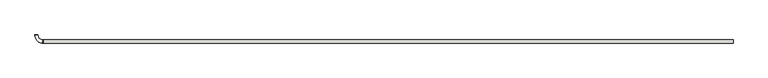
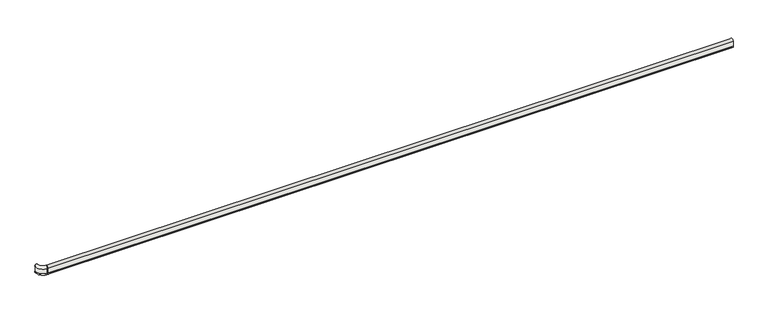
"""IFC4 building model written with IfcOpenShell, lengths in millimetres: covering geometry, Construction_Railing_SPM_Starline-Anodisee-Decowood : Decowood."""

from ifc_helpers import new_model, si_unit, point, frame, frame_2d, origin, place, context, project, spatial, polyline, circle_curve, ellipse_curve, trimmed, segment, composite_curve, outline, extrude, source, transform, mapped, element, save
from ifc_brep_helpers import plane_surface, cylinder_surface, revolved_surface, advanced_brep


def covering_4a841b85(model_context):
    return source(origin(), model_context, "Body", "SolidModel", [
        advanced_brep(
        [(0.0, -52.1949146, 777.1298269), (0.0, -78.97282, 779.8387167), (0.0, -77.7797808, 779.8387167), (0.0, -77.7797808, 730.187687), (0.0, -79.0444967, 730.187687), (0.0, -52.1949146, 732.7970729), (-1.0, -52.1949146, 777.1298269), (-1.0, -78.97282, 779.8387167), (-78.97282, -1.0, 779.8387167), (-78.97282, 0.0, 779.8387167), (-77.7797808, 0.0, 779.8387167), (-77.7797808, -1.0, 779.8387167), (-1.0, -77.7797808, 779.8387167), (-1.0, -77.7797808, 730.187687), (-77.7797808, -1.0, 730.187687), (-77.7797808, 0.0, 730.187687), (-79.0444967, 0.0, 730.187687), (-79.0444967, -1.0, 730.187687), (-1.0, -79.0444967, 730.187687), (-1.0, -52.1949146, 732.7970729), (-52.1949146, -1.0, 777.1298269), (-52.1949146, -1.0, 732.7970729), (-52.1949146, 0.0, 777.1298269), (-52.1949146, 0.0, 732.7970729)],
        [
            (0, 1, circle_curve(frame((0.0, -64.921376, 785.0331273), z_axis=(1.0, 0.0, 0.0), x_axis=(0.0, -1.0, 0.0)), 14.9808204)),
            (1, 2),
            (2, 3),
            (3, 4),
            (4, 5, circle_curve(frame((0.0, -64.9833199, 724.9442146), z_axis=(1.0, 0.0, 0.0), x_axis=(0.0, -1.0, 0.0)), 15.0070215)),
            (5, 0),
            (0, 6),
            (6, 7, circle_curve(frame((-1.0, -64.921376, 785.0331273), z_axis=(1.0, 0.0, 0.0), x_axis=(0.0, -1.0, 0.0)), 14.9808204)),
            (7, 1),
            (7, 8, circle_curve(frame((-1.0, -1.0, 779.8387167), z_axis=(0.0, 0.0, -1.0), x_axis=(0.0, -1.0, 0.0)), 77.97282)),
            (8, 9),
            (9, 10),
            (10, 11),
            (11, 12, circle_curve(frame((-1.0, -1.0, 779.8387167), z_axis=(0.0, 0.0, 1.0), x_axis=(0.0, -1.0, 0.0)), 76.7797808)),
            (12, 2),
            (12, 13),
            (13, 3),
            (13, 14, circle_curve(frame((-1.0, -1.0, 730.187687), z_axis=(0.0, 0.0, -1.0), x_axis=(0.0, -1.0, 0.0)), 76.7797808)),
            (14, 15),
            (15, 16),
            (16, 17),
            (17, 18, circle_curve(frame((-1.0, -1.0, 730.187687), z_axis=(0.0, 0.0, 1.0), x_axis=(0.0, -1.0, 0.0)), 78.0444967)),
            (18, 4),
            (18, 19, circle_curve(frame((-1.0, -64.9833199, 724.9442146), z_axis=(1.0, 0.0, 0.0), x_axis=(0.0, -1.0, 0.0)), 15.0070215)),
            (19, 5),
            (19, 6),
            (6, 20, circle_curve(frame((-1.0, -1.0, 777.1298269), z_axis=(0.0, 0.0, -1.0), x_axis=(0.0, -1.0, 0.0)), 51.1949146)),
            (20, 8, circle_curve(frame((-64.921376, -1.0, 785.0331273), z_axis=(0.0, -1.0, 0.0), x_axis=(-1.0, 0.0, 0.0)), 14.9808204)),
            (11, 14),
            (21, 19, circle_curve(frame((-1.0, -1.0, 732.7970729), z_axis=(0.0, 0.0, 1.0), x_axis=(0.0, -1.0, 0.0)), 51.1949146)),
            (17, 21, circle_curve(frame((-64.9833199, -1.0, 724.9442146), z_axis=(0.0, -1.0, 0.0), x_axis=(-1.0, 0.0, 0.0)), 15.0070215)),
            (21, 20),
            (22, 23),
            (23, 16, circle_curve(frame((-64.9833199, 0.0, 724.9442146), z_axis=(0.0, 1.0, 0.0), x_axis=(-1.0, 0.0, 0.0)), 15.0070215)),
            (15, 10),
            (9, 22, circle_curve(frame((-64.921376, 0.0, 785.0331273), z_axis=(0.0, 1.0, 0.0), x_axis=(-1.0, 0.0, 0.0)), 14.9808204)),
            (20, 22),
            (23, 21),
        ],
        [
            plane_surface(frame((0.0, -50.0, 710.0), z_axis=(1.0, 0.0, 0.0), x_axis=(0.0, 0.0, 1.0))),
            cylinder_surface(frame((0.0, -64.921376, 785.0331273), z_axis=(1.0, 0.0, 0.0), x_axis=(0.0, -1.0, 0.0)), 14.9808204),
            plane_surface(frame((0.0, -78.97282, 779.8387167), z_axis=(0.0, 0.0, -1.0), x_axis=(-1.0, 0.0, 0.0))),
            plane_surface(frame((0.0, -77.7797808, 779.8387167), z_axis=(0.0, -1.0, 0.0), x_axis=(-1.0, 0.0, 0.0))),
            plane_surface(frame((0.0, -77.7797808, 730.187687), z_axis=(0.0, 0.0, 1.0), x_axis=(-1.0, 0.0, 0.0))),
            cylinder_surface(frame((0.0, -64.9833199, 724.9442146), z_axis=(1.0, 0.0, 0.0), x_axis=(0.0, -1.0, 0.0)), 15.0070215),
            plane_surface(frame((0.0, -52.1949146, 732.7970729), z_axis=(0.0, 1.0, 0.0), x_axis=(-1.0, 0.0, 0.0))),
            revolved_surface(trimmed(ellipse_curve(frame((-1.0, -64.921376, 785.0331273), z_axis=(1.0, 0.0, 0.0), x_axis=(0.0, -1.0, 0.0)), 14.9808204, 14.9808204), [point((-1.0, -52.1949146, 777.1298269))], [point((-1.0, -78.97282, 779.8387167))], True, "CARTESIAN"), (-1.0, -1.0, 710.0), (0.0, 0.0, -1.0)),
            cylinder_surface(frame((-1.0, -1.0, 710.0), z_axis=(0.0, 0.0, -1.0), x_axis=(0.0, -1.0, 0.0)), 76.7797808),
            revolved_surface(trimmed(ellipse_curve(frame((-1.0, -64.9833199, 724.9442146), z_axis=(1.0, 0.0, 0.0), x_axis=(0.0, -1.0, 0.0)), 15.0070215, 15.0070215), [point((-1.0, -79.0444967, 730.187687))], [point((-1.0, -52.1949146, 732.7970729))], True, "CARTESIAN"), (-1.0, -1.0, 710.0), (0.0, 0.0, -1.0)),
            revolved_surface(polyline([(-1.0, -52.1949146, 732.7970729), (-1.0, -52.1949146, 777.1298269)]), (-1.0, -1.0, 710.0), (0.0, 0.0, -1.0)),
            plane_surface(frame((-50.0, 0.0, 710.0), z_axis=(0.0, 1.0, 0.0), x_axis=(0.0, 0.0, 1.0))),
            cylinder_surface(frame((-64.921376, -1.0, 785.0331273), z_axis=(0.0, -1.0, 0.0), x_axis=(-1.0, 0.0, 0.0)), 14.9808204),
            plane_surface(frame((-77.7797808, -1.0, 779.8387167), z_axis=(-1.0, 0.0, 0.0), x_axis=(0.0, 1.0, 0.0))),
            cylinder_surface(frame((-64.9833199, -1.0, 724.9442146), z_axis=(0.0, -1.0, 0.0), x_axis=(-1.0, 0.0, 0.0)), 15.0070215),
            plane_surface(frame((-52.1949146, -1.0, 732.7970729), z_axis=(1.0, 0.0, 0.0), x_axis=(0.0, 1.0, 0.0))),
        ],
        [
            (0, [[1, 2, 3, 4, 5, 6]]),
            (1, [[-1, 7, 8, 9]]),
            (2, [[-2, -9, 10, 11, 12, 13, 14, 15]]),
            (3, [[-3, -15, 16, 17]]),
            (4, [[-4, -17, 18, 19, 20, 21, 22, 23]]),
            (5, [[-5, -23, 24, 25]]),
            (6, [[-6, -25, 26, -7]]),
            (7, [[-10, -8, 27, 28]]),
            (8, [[-18, -16, -14, 29]]),
            (9, [[30, -24, -22, 31]]),
            (10, [[-27, -26, -30, 32]]),
            (11, [[33, 34, -20, 35, -12, 36]]),
            (12, [[-28, 37, -36, -11]]),
            (13, [[-29, -13, -35, -19]]),
            (14, [[-31, -21, -34, 38]]),
            (15, [[-32, -38, -33, -37]]),
        ],
    ),
        extrude(outline(composite_curve([segment(trimmed(circle_curve(frame_2d((-64.921376, 785.0331273)), 14.9808204), [point((-78.97282, 779.8387167))], [point((-52.1949146, 777.1298269))], False, "CARTESIAN"), True, "CONTINUOUS"), segment(polyline([(-52.1949146, 777.1298269), (-52.1949146, 732.7970729)]), True, "CONTINUOUS"), segment(trimmed(circle_curve(frame_2d((-64.9833199, 724.9442146)), 15.0070215), [point((-52.1949146, 732.7970729))], [point((-79.0444967, 730.187687))], False, "CARTESIAN"), True, "CONTINUOUS"), segment(polyline([(-79.0444967, 730.187687), (-77.7797808, 730.187687), (-77.7797808, 779.8387167), (-78.97282, 779.8387167)]), True, "CONTINUOUS")], self_intersect=False)), frame((0.0, 0.0, 0.0), z_axis=(1.0, 0.0, 0.0), x_axis=(0.0, 1.0, 0.0)), (0.0, 0.0, 1.0), 6800.0),
        extrude(outline(polyline([(0.0, -79.3173438), (0.0, -77.7797808), (6800.0, -77.7797808), (6800.0, -79.3173438), (0.0, -79.3173438)])), frame((0.0, 0.0, 730.187687), z_axis=(0.0, 0.0, 1.0), x_axis=(1.0, 0.0, 0.0)), (0.0, 0.0, 1.0), 49.6510297),
    ])


if __name__ == "__main__":
    model = new_model("IFC4")
    model_context = context("Model", 3, world=origin())
    ifc_project = project(units=[si_unit("LENGTHUNIT", "METRE", prefix="MILLI")], contexts=[model_context])
    site = spatial("IfcSite", under=ifc_project)
    building = spatial("IfcBuilding", under=site)
    placement = place(None, origin())
    covering_shape = covering_4a841b85(model_context)
    element("IfcCovering", 1, ObjectType="Construction_Railing_SPM_Starline-Anodisee-Decowood : Decowood", at=placement, inside=building, context=model_context, shape_type="MappedRepresentation", body=[
        mapped(covering_shape, transform((0.0, 0.0, 0.0), x_axis=(1.0, 0.0, 0.0), y_axis=(0.0, 1.0, 0.0), z_axis=(0.0, 0.0, 1.0))),
    ])
    save(model, "model.ifc")

# Revit data of these elements
# Type "Construction_Railing_SPM_Starline-Anodisee-Decowood : Decowood"
#   WarrantyStartDate [instance default] = "1900-12-31T23:59:59"
#   WarrantyGuarantorParts = "n/a"
#   WarrantyGuarantorLabor = "n/a"
#   WarrantyDurationUnit = "year"
#   WarrantyDurationParts = "n/a"
#   WarrantyDurationLabor = "n/a"
#   WarrantyDescription = "n/a"
#   WallStandoff = "50 mm"
#   URL = "www.spm.fr"
#   UNSPSC Code = ""
#   TagNumber [instance default] = "n/a"
#   SustainabilityPerformance = "n/a"
#   SurfaceSpreadOfFlame = "n/a"
#   Size = "90 x 80 x 4000 mm"
#   Shape = "Elliptical"
#   SerialNumber [instance default] = "n/a"
#   ReplacementCost = "n/a"
#   Reference = "n/a"
#   Projection = "80 mm"
#   Product data url = "http://bimobject.com/spm/product/SPM-STARLINE-DECO"
#   Product Guid = "a7a4224a-4578-432f-a478-06146786615d"
#   OmniClass Description = ""
#   OmniClass Code = ""
#   Name = "WallProtectionPanels_StarlineDecowoodHandrail_GerflorLtd"
#   NBS Reference Description = ""
#   NBS Reference Code = ""
#   ModelReference = "Starline Decowood Handrail"
#   ModelNumber = "n/a"
#   Model = "Starline Decowood Handrail"
#   Material secondary = ""
#   Material main = ""
#   Material = "1.5 mm thick aluminium"
#   Manufacturer = "SPM"
#   Keynote = "09100"
#   InstallationDate [instance default] = "1900-12-31T23:59:59"
#   IfcExportType = "NOTDEFINED"
#   IfcExportAs = "IfcCoveringType"
#   IFC Classification = ""
#   Grade = "n/a"
#   FragilityRating = "n/a"
#   FlammabilityRating = "n/a"
#   Fixing = "2-point self-locking perforated satin silver anodized aluminium brackets"
#   FireRating = "B-s2, d0"
#   Finish = "Aluminium profile: Satin silver anodized; PVC band: Wood effect"
#   Features = "Excellent wrenching resistance, antibacterial"
#   ExpectedLife = "n/a"
#   EnvironmentalProductDeclaration = "n/a"
#   EAN code = ""
#   DurationUnit = "year"
#   Description = "Range only available for the French market"
#   CrossSection = "Elliptical"
#   Constituents = "n/a"
#   ColourOptions = "PVC band: 7 wood effect and 2 trend effect colours available"
#   Color = "n/a"
#   CodePerformance = "n/a"
#   Category = "n/a"
#   COBIe Type Category = ""
#   BarCode [instance default] = "n/a"
#   BIMobject category = ""
#   AssetType = "Fixed"
#   AssetIdentifier [instance default] = "n/a"
#   Assembly Code = "C10"
#   Applications = "Straight and curved corridors in public buildings such as hospitals, clinics, retirement homes, hotels and offices"
#   AcousticRating = "n/a"
#   Accessories = "90° external angle pieces, Variable angles, Wall returns"
#   AccessibilityPerformance = "n/a"
#   Width = 80 mm
#   TotalThickness = 80 mm
#   SpacerOffsetRight [instance default] = 100 mm
#   SpacerOffsetLeft [instance default] = 100 mm
#   OffsetFromWall = 50 mm
#   NominalLength [instance default] = 4000 mm
#   Height = 90 mm
#   HandrailHeight [instance default] = 800 mm
#   SpacerVerticalPlacement [instance default] = 724 mm
#   SpacerCentreToCentreDistance [instance default] = 950 mm
#   SpacerCalc [instance default] = 3800 mm
#   SpacerOffsetRightControl [instance default] = 100 mm
#   SpacerOffsetLeftControl [instance default] = 100 mm
#   MaximumSpacerCentreDistance [instance default] = 1200 mm
#   built-in parameter 1001306 [instance default] = 13.1234 (stored number, unit not read)
#   Diameter = 0 mm
#   Depth = 80 mm
#   NumberOfStandardRailLengths [instance default] = 1
#   NumberOfSpacers [instance default] = 5
#   IsExternal = no
#   HasHeavyTraffic [instance default] = no
#   Edition number = 1
#   CrashRailInternalCornerRight [instance default] = no
#   CrashRailInternalCornerLeft [instance default] = no
#   CrashRailExternalCornerRight [instance default] = yes
#   CrashRailExternalCornerLeft [instance default] = yes
#   CrashRailEndCapRight [instance default] = no
#   CrashRailEndCapLeft [instance default] = no
#   Combustible = no
#   InsertMaterial = PVC - SPM - Erable
#   SpacerMaterial = PVC - SPM - Hêtre
#   RailMaterial = PVC - SPM - Wengé
#   Default Elevation = 0
#   Cost = 0
# Element 1 (IfcCovering, "Construction_Railing_SPM_Starline-Anodisee-Decowood : Decowood")
#   NominalLength = 6800 mm
#   SpacerCentreToCentreDistance = 1100 mm
#   SpacerCalc = 6600 mm
#   built-in parameter 1001306 = 22.3097 (stored number, unit not read)
#   NumberOfStandardRailLengths = 2
#   NumberOfSpacers = 7
#   Materials on its faces: "PVC - SPM - Wengé", "PVC - SPM - Erable"
# Materials
#   "PVC - SPM - Erable": class "Plastique", colour RGB 155 148 134, transparency 0, Keynote = "09700", Model = "0060 Erable", Manufacturer = "SPM", URL = "www.spm.fr", Description = "Gamme Bois", Cost = 0
#   "PVC - SPM - Hêtre": class "Plastique", colour RGB 140 126 100, transparency 0, Keynote = "09700", Model = "0061 Hêtre", Manufacturer = "SPM", URL = "www.spm.fr", Description = "Gamme Bois", Cost = 0
#   "PVC - SPM - Wengé": class "Plastique", colour RGB 64 50 47, transparency 0, Keynote = "09700", Model = "0067 Wengé", Manufacturer = "SPM", URL = "www.spm.fr", Description = "Gamme Bois", Cost = 0
